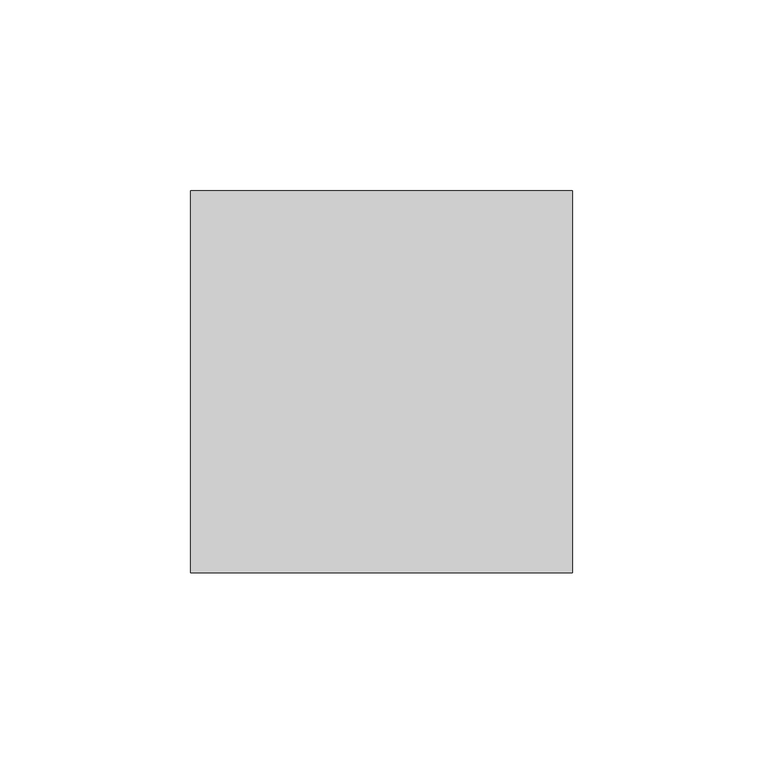
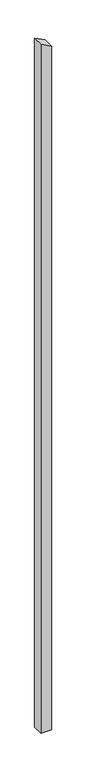
"""IFC4 building model written with IfcOpenShell, lengths in millimetres: column geometry, Holzstütze 159256 : Holzstütze 159256."""

from ifc_helpers import new_model, si_unit, frame, origin, place, context, project, spatial, polyline, outline, extrude, source, transform, mapped, element, save


def column_b6b0c2fc(model_context):
    return source(origin(), model_context, "Body", "SweptSolid", [
        extrude(outline(polyline([(-500.0, 174197.7593015), (-500.0, 174297.7593015), (6345.7118258, 174297.7593015), (6396.6643707, 174197.7593015), (-500.0, 174197.7593015)])), frame((0.0, 36959.3988814, 0.0), z_axis=(0.0, 1.0, 0.0), x_axis=(0.0, 0.0, 1.0)), (0.0, 0.0, 1.0), 100.0),
    ])


if __name__ == "__main__":
    model = new_model("IFC4")
    model_context = context("Model", 3, world=origin())
    ifc_project = project(units=[si_unit("LENGTHUNIT", "METRE", prefix="MILLI")], contexts=[model_context])
    site = spatial("IfcSite", under=ifc_project)
    building = spatial("IfcBuilding", under=site)
    placement = place(None, origin())
    column_shape = column_b6b0c2fc(model_context)
    element("IfcColumn", 1, ObjectType="Holzstütze 159256 : Holzstütze 159256", at=placement, inside=building, context=model_context, shape_type="MappedRepresentation", body=[
        mapped(column_shape, transform((0.0, 0.0, 0.0), x_axis=(1.0, 0.0, 0.0), y_axis=(0.0, 1.0, 0.0), z_axis=(0.0, 0.0, 1.0))),
    ])
    save(model, "model.ifc")

# Revit data of these elements
# Type "Holzstütze 159256 : Holzstütze 159256"
#   Abrechnungsart = "m"
#   Allright_Bauteil_ID = "0152St 0000143356"
#   Bezeichnung = "Holzstütze"
#   Codetext = "ST-HOLZ\\"
#   Gewerk = "Zimmer- und Holzbauarbeiten"
#   Material = "Holz"
#   Objektname = "Stütze"
#   NameOverride = "Holzstütze"
#   Reference = "Holzstütze"
#   Status = "NEW"
#   ThermalTransmittance = 0.0000 BTU/(h·ft²·°F)
#   Roll = 0.00°
#   Slope = 0.00°
#   2D Interaktion = yes
#   IsExternal = yes
#   LoadBearing = yes
# Element 1 (IfcColumn, "Holzstütze 159256 : Holzstütze 159256")
#   Materials on its faces: "holzschalung"
# Materials
#   "holzschalung": class "Unassigned", colour RGB 128 128 128, transparency 0
